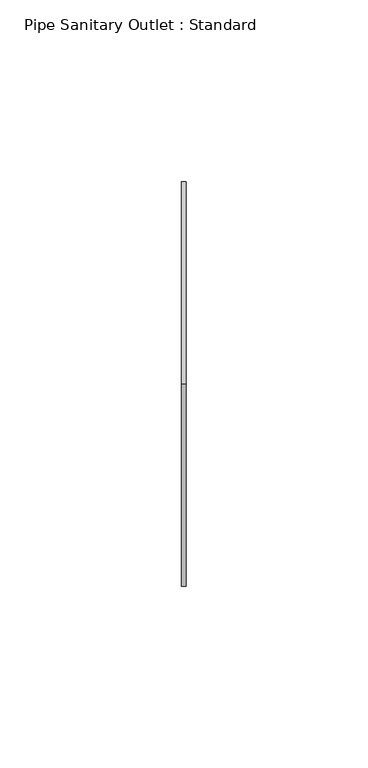
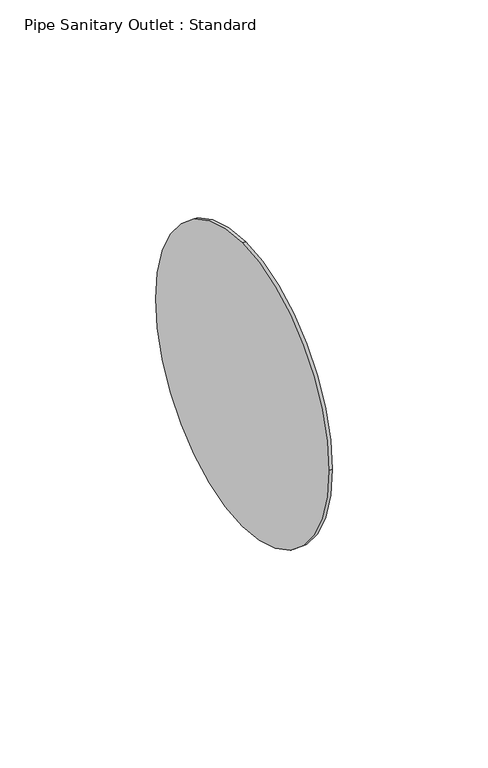
"""IFC4 building model written with IfcOpenShell, lengths in millimetres: proxy geometry, Pipe Sanitary Outlet : Standard."""

from ifc_helpers import new_model, si_unit, point, frame, origin, origin_2d, place, context, project, spatial, circle_curve, trimmed, segment, composite_curve, outline, extrude, source, transform, mapped, element, save


def pipe_sanitary_outlet_standard_9883e289(model_context):
    return source(origin(), model_context, "Body", "SweptSolid", [
        extrude(outline(composite_curve([segment(trimmed(circle_curve(origin_2d(), 55.5625), [point((0.0, 55.5625))], [point((55.5625, 0.0))], False, "CARTESIAN"), True, "CONTINUOUS"), segment(trimmed(circle_curve(origin_2d(), 55.5625), [point((55.5625, 0.0))], [point((0.0, -55.5625))], False, "CARTESIAN"), True, "CONTINUOUS"), segment(trimmed(circle_curve(origin_2d(), 55.5625), [point((0.0, -55.5625))], [point((-55.5625, 0.0))], False, "CARTESIAN"), True, "CONTINUOUS"), segment(trimmed(circle_curve(origin_2d(), 55.5625), [point((-55.5625, 0.0))], [point((0.0, 55.5625))], False, "CARTESIAN"), True, "CONTINUOUS")], self_intersect=False)), frame((0.0, 0.0, 0.0), z_axis=(1.0, 0.0, 0.0), x_axis=(0.0, 1.0, 0.0)), (0.0, 0.0, 1.0), 1.27),
        extrude(outline(composite_curve([segment(trimmed(circle_curve(origin_2d(), 55.5625), [point((0.0, 55.5625))], [point((55.5625, 0.0))], False, "CARTESIAN"), True, "CONTINUOUS"), segment(trimmed(circle_curve(origin_2d(), 55.5625), [point((55.5625, 0.0))], [point((0.0, -55.5625))], False, "CARTESIAN"), True, "CONTINUOUS"), segment(trimmed(circle_curve(origin_2d(), 55.5625), [point((0.0, -55.5625))], [point((-55.5625, 0.0))], False, "CARTESIAN"), True, "CONTINUOUS"), segment(trimmed(circle_curve(origin_2d(), 55.5625), [point((-55.5625, 0.0))], [point((0.0, 55.5625))], False, "CARTESIAN"), True, "CONTINUOUS")], self_intersect=False)), frame((0.0, 0.0, 0.0), z_axis=(1.0, 0.0, 0.0), x_axis=(0.0, 1.0, 0.0)), (0.0, 0.0, 1.0), 1.27),
    ])


if __name__ == "__main__":
    model = new_model("IFC4")
    model_context = context("Model", 3, world=origin())
    ifc_project = project(units=[si_unit("LENGTHUNIT", "METRE", prefix="MILLI")], contexts=[model_context])
    site = spatial("IfcSite", under=ifc_project)
    building = spatial("IfcBuilding", under=site)
    placement = place(None, origin())
    pipe_sanitary_outlet_standard_shape = pipe_sanitary_outlet_standard_9883e289(model_context)
    element("IfcBuildingElementProxy", 1, Name="Pipe Sanitary Outlet : Standard", ObjectType="Pipe Sanitary Outlet : Standard", at=placement, inside=building, context=model_context, shape_type="MappedRepresentation", body=[
        mapped(pipe_sanitary_outlet_standard_shape, transform((0.0, 0.0, 0.0), x_axis=(1.0, 0.0, 0.0), y_axis=(0.0, 1.0, 0.0), z_axis=(0.0, 0.0, 1.0))),
    ])
    save(model, "model.ifc")

# Revit data of these elements
# Type "Pipe Sanitary Outlet : Standard"
#   Lookup Table Name [instance default] = "Pipe Fitting Sizes"
#   WaterFlow [instance default] = 0 GPM
#   Radius [instance default] = 2 3/16"
#   Nominal Size [instance default] = 4"
#   Nominal Radius [instance default] = 2"
#   Insulation Thickness [instance default] = 0"
#   Insulation Radius [instance default] = 2 3/16"
#   IsCustom [instance default] = no
#   Assembly Code = ""
